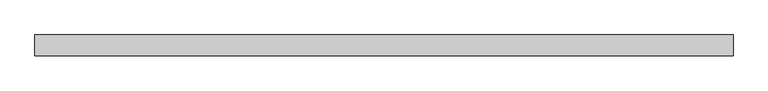
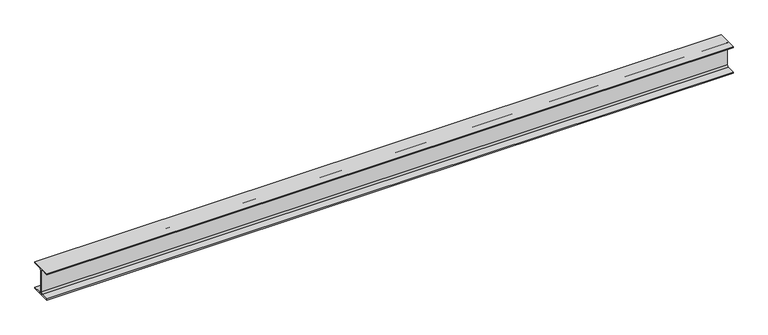
"""IFC4 building model written with IfcOpenShell, lengths in millimetres: beam geometry, 0912_Steel Framing_H-KSD3502 : H_SB_ASB_H-340x250x9x14."""

import ifcopenshell
import ifcopenshell.guid

model = None  # the IFC model being written
_history = None  # IfcOwnerHistory: only IFC2X3 demands one
_inside = {}  # id of a spatial element -> (the spatial element, [elements in it])
_under = {}  # id of a project, library or spatial element -> (it, [spatial elements below it])
_declared = {}  # id of a project -> (the project, [libraries it declares])
_typed = {}  # id of a type object -> (the type object, [elements of that type])
_made_of = {}  # id of a material, layer set ... -> (it, [elements and type objects made of it])


def new_model(schema):
    """Start an empty IFC model of exactly this schema.

    Asked for "IFC4X3", IfcOpenShell would pick the latest addendum, in which some entities
    have other attributes; the version numbers below select the first issue.
    IFC2X3 requires an IfcOwnerHistory on every rooted entity: one is made here for all.
    """
    global model, _history
    if schema == "IFC4X3":
        model = ifcopenshell.file(schema_version=(4, 3, 0, 0))
    else:
        model = ifcopenshell.file(schema=schema)
    _inside.clear()
    _under.clear()
    _declared.clear()
    _typed.clear()
    _made_of.clear()
    _history = None
    if model.schema == "IFC2X3":
        org = make("IfcOrganization", Name="unknown")
        user = make(
            "IfcPersonAndOrganization",
            ThePerson=make("IfcPerson", FamilyName="unknown"),
            TheOrganization=org,
        )
        app = make(
            "IfcApplication",
            ApplicationDeveloper=org,
            Version="unknown",
            ApplicationFullName="unknown",
            ApplicationIdentifier="unknown",
        )
        _history = make(
            "IfcOwnerHistory",
            OwningUser=user,
            OwningApplication=app,
            ChangeAction="ADDED",
            CreationDate=0,
        )
    return model


def make(cls, **values):
    """One entity of the class cls with the attributes given. An attribute that is None is left unset."""
    return model.create_entity(
        cls, **{name: value for name, value in values.items() if value is not None}
    )


def rooted(cls, **values):
    """An entity with a GlobalId (a new one), such as an element, a storey or a relation."""
    return make(cls, GlobalId=ifcopenshell.guid.new(), OwnerHistory=_history, **values)


def si_unit(unit_type, name, prefix=None):
    """IfcSIUnit, for example si_unit("LENGTHUNIT", "METRE", prefix="MILLI")."""
    return make("IfcSIUnit", UnitType=unit_type, Prefix=prefix, Name=name)


def assignment(units):
    """IfcUnitAssignment: the units of a project."""
    return None if units is None else make("IfcUnitAssignment", Units=units)


def point(xyz):
    """IfcCartesianPoint."""
    return None if xyz is None else make("IfcCartesianPoint", Coordinates=xyz)


def direction(xyz):
    """IfcDirection."""
    return None if xyz is None else make("IfcDirection", DirectionRatios=xyz)


def frame(location, z_axis=None, x_axis=None):
    """IfcAxis2Placement3D, a coordinate frame: its origin and axes. An axis left out is left unset."""
    return make(
        "IfcAxis2Placement3D",
        Location=point(location),
        Axis=direction(z_axis),
        RefDirection=direction(x_axis),
    )


def frame_2d(location, x_axis=None):
    """IfcAxis2Placement2D, a coordinate frame in the plane: its origin and x axis."""
    return make(
        "IfcAxis2Placement2D", Location=point(location), RefDirection=direction(x_axis)
    )


def origin():
    """The frame at (0, 0, 0) with its axes left unset."""
    return frame((0.0, 0.0, 0.0))


def place(relative_to, where):
    """IfcLocalPlacement: puts the frame where relative to a parent placement (None: the world)."""
    return make(
        "IfcLocalPlacement", PlacementRelTo=relative_to, RelativePlacement=where
    )


def context(
    kind, dimensions, precision=None, world=None, true_north=None, identifier=None
):
    """IfcGeometricRepresentationContext, for example the 3D "Model" context."""
    return make(
        "IfcGeometricRepresentationContext",
        ContextIdentifier=identifier,
        ContextType=kind,
        CoordinateSpaceDimension=dimensions,
        Precision=precision,
        WorldCoordinateSystem=world,
        TrueNorth=true_north,
    )


def project(units=None, contexts=None):
    """IfcProject with its units and contexts."""
    return rooted(
        "IfcProject",
        Name="project",
        RepresentationContexts=contexts,
        UnitsInContext=assignment(units),
    )


def spatial(cls, under=None, at=None, **own):
    """A site, building, storey or space (cls), placed at a placement, below another one or the project."""
    s = rooted(cls, ObjectPlacement=at, **own)
    if under is not None:
        _under.setdefault(under.id(), (under, []))[1].append(s)
    return s


def polyline(points):
    """IfcPolyline through the points."""
    return make("IfcPolyline", Points=[point(p) for p in points])


def circle_curve(where, radius):
    """IfcCircle in the frame where."""
    return make("IfcCircle", Position=where, Radius=radius)


def trimmed(basis, trim1, trim2, sense, master):
    """IfcTrimmedCurve: the piece of a basis curve between two trims."""
    return make(
        "IfcTrimmedCurve",
        BasisCurve=basis,
        Trim1=trim1,
        Trim2=trim2,
        SenseAgreement=sense,
        MasterRepresentation=master,
    )


def segment(curve, same_sense, transition):
    """IfcCompositeCurveSegment."""
    return make(
        "IfcCompositeCurveSegment",
        Transition=transition,
        SameSense=same_sense,
        ParentCurve=curve,
    )


def composite_curve(segments, self_intersect=None):
    """IfcCompositeCurve: segments joined end to end."""
    return make("IfcCompositeCurve", Segments=segments, SelfIntersect=self_intersect)


def outline(outer, holes=None, kind="AREA"):
    """IfcArbitraryClosedProfileDef: a profile drawn as a closed curve; with holes, ...WithVoids."""
    if holes is None:
        return make("IfcArbitraryClosedProfileDef", ProfileType=kind, OuterCurve=outer)
    return make(
        "IfcArbitraryProfileDefWithVoids",
        ProfileType=kind,
        OuterCurve=outer,
        InnerCurves=holes,
    )


def extrude(swept, where, along, depth):
    """IfcExtrudedAreaSolid: the profile swept, set in the frame where, extruded along a direction by depth."""
    return make(
        "IfcExtrudedAreaSolid",
        SweptArea=swept,
        Position=where,
        ExtrudedDirection=direction(along),
        Depth=depth,
    )


def shape(context_of_items, identifier, shape_type, items):
    """IfcShapeRepresentation: the items that make up one representation, for example the "Body"."""
    return make(
        "IfcShapeRepresentation",
        ContextOfItems=context_of_items,
        RepresentationIdentifier=identifier,
        RepresentationType=shape_type,
        Items=items,
    )


def source(mapping_origin, context_of_items, identifier, shape_type, items):
    """IfcRepresentationMap: a shape defined once, which mapped items show again and again."""
    return make(
        "IfcRepresentationMap",
        MappingOrigin=mapping_origin,
        MappedRepresentation=shape(context_of_items, identifier, shape_type, items),
    )


def transform(
    local_origin,
    x_axis=None,
    y_axis=None,
    z_axis=None,
    scale=None,
    scale2=None,
    scale3=None,
    uniform=True,
):
    """IfcCartesianTransformationOperator3D, or its non-uniform kind. x_axis, y_axis, z_axis: its Axis1, 2, 3."""
    if uniform:
        return make(
            "IfcCartesianTransformationOperator3D",
            Axis1=direction(x_axis),
            Axis2=direction(y_axis),
            LocalOrigin=point(local_origin),
            Scale=scale,
            Axis3=direction(z_axis),
        )
    return make(
        "IfcCartesianTransformationOperator3DnonUniform",
        Axis1=direction(x_axis),
        Axis2=direction(y_axis),
        LocalOrigin=point(local_origin),
        Scale=scale,
        Axis3=direction(z_axis),
        Scale2=scale2,
        Scale3=scale3,
    )


def mapped(mapping_source, mapping_target):
    """IfcMappedItem: shows the shape of a source again, moved by a transform."""
    return make(
        "IfcMappedItem", MappingSource=mapping_source, MappingTarget=mapping_target
    )


def made_of(thing, what):
    """Note that an element or type object is made of a material, layer set ...; save() writes the relation."""
    if what is not None:
        _made_of.setdefault(what.id(), (what, []))[1].append(thing)
    return thing


def element(
    cls,
    number,
    at=None,
    inside=None,
    cuts=None,
    type_object=None,
    material=None,
    context=None,
    identifier="Body",
    shape_type=None,
    held_by="IfcProductDefinitionShape",
    body=None,
    shapes=None,
    **own,
):
    """One element of the class cls, such as IfcWall. Its Tag is "e" and its number.

    at: its placement. inside: the storey or other place that contains it. cuts: it is an
    opening in that element (IfcRelVoidsElement). A single representation is given by context,
    identifier, shape_type and body (its items); several are given by shapes. held_by: the class
    of the entity that holds the representations. save() writes the other relations.
    """
    e = rooted(cls, Tag="e%d" % number, ObjectPlacement=at, **own)
    if body is not None:
        shapes = [shape(context, identifier, shape_type, body)]
    if shapes is not None:
        e.Representation = make(held_by, Representations=shapes)
    if inside is not None:
        _inside.setdefault(inside.id(), (inside, []))[1].append(e)
    if cuts is not None:
        rooted(
            "IfcRelVoidsElement", RelatingBuildingElement=cuts, RelatedOpeningElement=e
        )
    if type_object is not None:
        _typed.setdefault(type_object.id(), (type_object, []))[1].append(e)
    return made_of(e, material)


def aggregate(whole, parts):
    """IfcRelAggregates: a whole, such as a stair, and the parts it consists of."""
    return rooted("IfcRelAggregates", RelatingObject=whole, RelatedObjects=parts)


def save(model, path):
    """Write the relations noted so far, then the file.

    IfcRelAggregates (storeys below a building ...), IfcRelContainedInSpatialStructure (elements
    in a storey), IfcRelDefinesByType, IfcRelAssociatesMaterial and IfcRelDeclares: one each for
    every whole, place, type object, material and project.
    """
    for whole, parts in _under.values():
        aggregate(whole, parts)
    for where, things in _inside.values():
        rooted(
            "IfcRelContainedInSpatialStructure",
            RelatedElements=things,
            RelatingStructure=where,
        )
    for kind, things in _typed.values():
        rooted("IfcRelDefinesByType", RelatedObjects=things, RelatingType=kind)
    for what, things in _made_of.values():
        rooted("IfcRelAssociatesMaterial", RelatedObjects=things, RelatingMaterial=what)
    for by, libraries in _declared.values():
        rooted("IfcRelDeclares", RelatingContext=by, RelatedDefinitions=libraries)
    model.write(path)


def beam_f474a5f9(model_context):
    return source(origin(), model_context, "Body", "SweptSolid", [
        extrude(outline(composite_curve([segment(polyline([(125.0, -156.0), (125.0, -170.0), (-125.0, -170.0), (-125.0, -156.0), (-24.5, -156.0)]), True, "CONTINUOUS"), segment(trimmed(circle_curve(frame_2d((-24.5, -136.0)), 20.0), [point((-24.5, -156.0))], [point((-4.5, -136.0))], True, "CARTESIAN"), True, "CONTINUOUS"), segment(polyline([(-4.5, -136.0), (-4.5, 136.0)]), True, "CONTINUOUS"), segment(trimmed(circle_curve(frame_2d((-24.5, 136.0)), 20.0), [point((-4.5, 136.0))], [point((-24.5, 156.0))], True, "CARTESIAN"), True, "CONTINUOUS"), segment(polyline([(-24.5, 156.0), (-125.0, 156.0), (-125.0, 170.0), (125.0, 170.0), (125.0, 156.0), (24.5, 156.0)]), True, "CONTINUOUS"), segment(trimmed(circle_curve(frame_2d((24.5, 136.0)), 20.0), [point((24.5, 156.0))], [point((4.5, 136.0))], True, "CARTESIAN"), True, "CONTINUOUS"), segment(polyline([(4.5, 136.0), (4.5, -136.0)]), True, "CONTINUOUS"), segment(trimmed(circle_curve(frame_2d((24.5, -136.0)), 20.0), [point((4.5, -136.0))], [point((24.5, -156.0))], True, "CARTESIAN"), True, "CONTINUOUS"), segment(polyline([(24.5, -156.0), (125.0, -156.0)]), True, "CONTINUOUS")], self_intersect=False)), frame((-4154.8, 0.0, 0.0), z_axis=(1.0, 0.0, 0.0), x_axis=(0.0, 1.0, 0.0)), (0.0, 0.0, 1.0), 8309.6),
    ])


if __name__ == "__main__":
    model = new_model("IFC4")
    model_context = context("Model", 3, world=origin())
    ifc_project = project(units=[si_unit("LENGTHUNIT", "METRE", prefix="MILLI")], contexts=[model_context])
    site = spatial("IfcSite", under=ifc_project)
    building = spatial("IfcBuilding", under=site)
    placement = place(None, origin())
    beam_shape = beam_f474a5f9(model_context)
    element("IfcBeam", 1, ObjectType="0912_Steel Framing_H-KSD3502 : H_SB_ASB_H-340x250x9x14", at=placement, inside=building, context=model_context, shape_type="MappedRepresentation", body=[
        mapped(beam_shape, transform((0.0, 0.0, 0.0), x_axis=(1.0, 0.0, 0.0), y_axis=(0.0, 1.0, 0.0), z_axis=(0.0, 0.0, 1.0))),
    ])
    save(model, "model.ifc")

# Revit data of these elements
# Type "0912_Steel Framing_H-KSD3502 : H_SB_ASB_H-340x250x9x14"
#   H_WM Code_1 = "S01AA002-00001 | Main Steel Structure Fabrication Work | Shelter/Building | Medium Steel - Standard (90KG/M>Weight≥30KG/M) | Material: (   )"
#   H_WM Code_2 = "S03AA028-00001 | Main Steel Structure Erection Work | Shelter/Building | Medium Steel (90KG/M>Weight≥30KG/M) | Material: (   )"
#   H_WM Code_3 = "S01AA010-00001 | Main Steel Structure Fabrication Work | Shelter/Building | Steel Painting/Coating | for Non-Fireproofed Steel Surface, Surface Preparation, Primer, Second & Final Coat | Material: (   )"
#   H_Q'ty Cal Type Tag = "SB-Q2"
#   Width = 25.0 cm
#   Web Thickness = 0.9 cm
#   Web Fillet = 2.0 cm
#   Warping Constant = 969000.0 cm⁶
#   W = 0
#   Torsional Moment of Inertia = 53.6551 cm⁴
#   Section Area = 101.5 cm²
#   Plastic Modulus weak axis = 447.0 cm³
#   Plastic Modulus strong axis = 1410.0 cm³
#   Perimeter = 1.63 m²/m
#   Nominal Weight = 79.70 kgf/m
#   Moment of Inertia weak axis = 3650.00 cm⁴
#   Moment of Inertia strong axis = 21700.00 cm⁴
#   Height = 34.0 cm
#   Flange Thickness = 1.4 cm
#   Elastic Modulus weak axis = 292.0 cm³
#   Elastic Modulus strong axis = 1280.0 cm³
#   Centroid Vertical = 17.0 cm
#   Centroid Horizontal = 12.5 cm
#   Ix = 217000000
#   Length [instance default] = 1.5240 m
#   Zx = 1410000
#   b = 0.2500 m
#   h = 0.3400 m
#   r = 0.0200 m
#   s = 0.0090 m
#   t = 0.0140 m
#   A = 0.01015 m²
#   Structural Material [instance default] = Steel, 45-345
#   Assembly Code = ""
# Element 1 (IfcBeam, "0912_Steel Framing_H-KSD3502 : H_SB_ASB_H-340x250x9x14")
#   Structural Material = none
# Materials
#   "Steel, 45-345": class "Metal", colour RGB 189 187 185, transparency 0, Description = "Steel 345 MPa", Cost = 0
